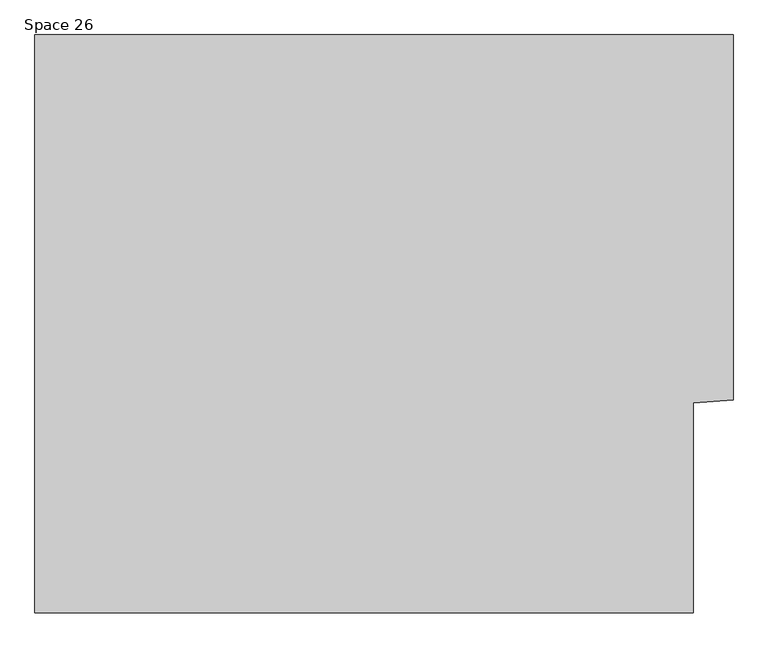
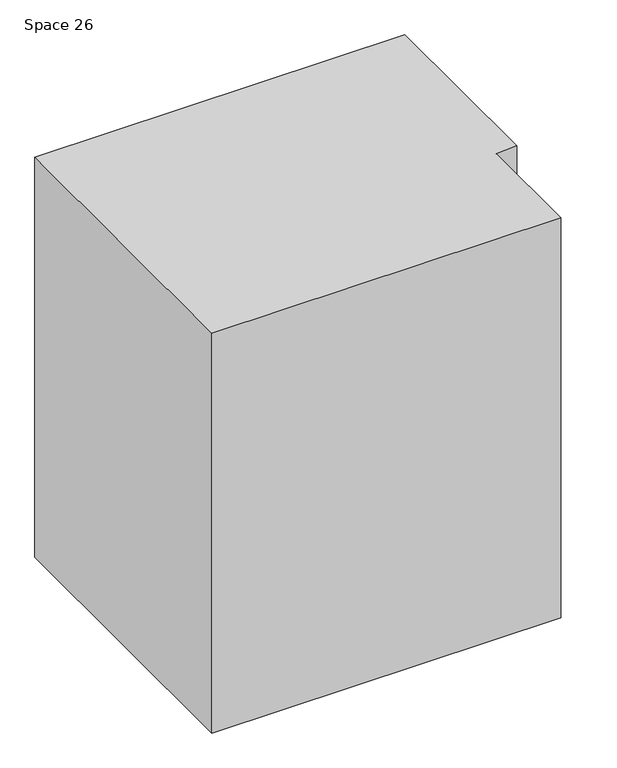
"""IFC4 building model written with IfcOpenShell, lengths in millimetres: proxy geometry, Space 26."""

from ifc_helpers import new_model, si_unit, origin, origin_with_axes, place, context, project, spatial, polyline, outline, extrude, source, transform, mapped, element, save


def space_26_e584359f(model_context):
    return source(origin(), model_context, "Body", "SweptSolid", [
        extrude(outline(polyline([(3148.0559655, -16439.359635), (5815.0559655, -16439.359635), (5815.0559655, -17835.3559389), (5662.6559655, -17846.012785), (5662.6559655, -18649.159635), (3148.0559655, -18649.159635), (3148.0559655, -16439.359635)])), origin_with_axes(), (0.0, 0.0, 1.0), 3048.0),
    ])


if __name__ == "__main__":
    model = new_model("IFC4")
    model_context = context("Model", 3, world=origin())
    ifc_project = project(units=[si_unit("LENGTHUNIT", "METRE", prefix="MILLI")], contexts=[model_context])
    site = spatial("IfcSite", under=ifc_project)
    building = spatial("IfcBuilding", under=site)
    placement = place(None, origin())
    space_26_shape = space_26_e584359f(model_context)
    element("IfcBuildingElementProxy", 1, Name="Space 26", ObjectType="Space 26", at=placement, inside=building, context=model_context, shape_type="MappedRepresentation", body=[
        mapped(space_26_shape, transform((0.0, 0.0, 0.0), x_axis=(1.0, 0.0, 0.0), y_axis=(0.0, 1.0, 0.0), z_axis=(0.0, 0.0, 1.0))),
    ])
    save(model, "model.ifc")

# Revit data of these elements
# Element 1 (IfcBuildingElementProxy, "Space 26")
#   Materials on its faces: "Render Material 255-255-255"
# Materials
#   "Render Material 255-255-255": class "Unassigned", colour RGB 255 255 255, transparency 0
